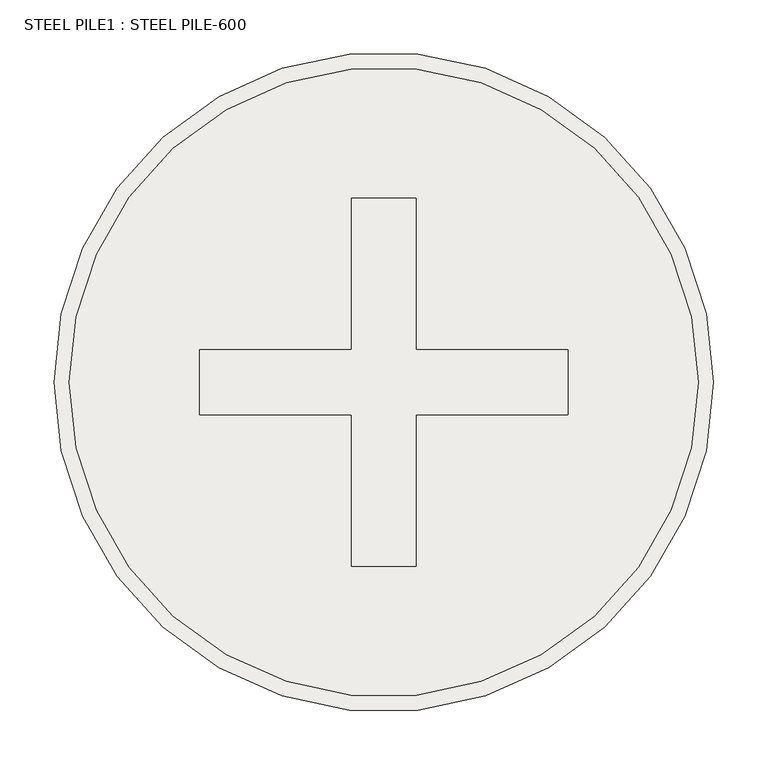
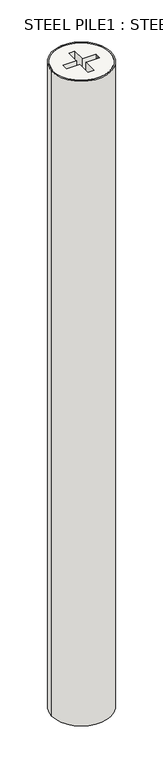
"""IFC4 building model written with IfcOpenShell, lengths in millimetres: slab geometry, STEEL PILE1 : STEEL PILE-600."""

from ifc_helpers import new_model, si_unit, point, frame, frame_2d, origin, place, context, project, spatial, circle_curve, trimmed, segment, composite_curve, outline, extrude, source, transform, mapped, element, save
from ifc_brep_helpers import plane_surface, cylinder_surface, advanced_brep


def steel_pile1_steel_pile_600_91f59ebf(model_context):
    return source(origin(), model_context, "Body", "SolidModel", [
        advanced_brep(
        [(-290.5, 22499.5208589, 150.0), (290.5, 22499.5208589, 150.0), (-30.0, 22469.5208589, 150.0), (-170.0, 22469.5208589, 150.0), (-170.0, 22499.5208589, 150.0), (-170.0, 22529.5208589, 150.0), (-30.0, 22529.5208589, 150.0), (-30.0, 22669.5208589, 150.0), (30.0, 22669.5208589, 150.0), (30.0, 22529.5208589, 150.0), (170.0, 22529.5208589, 150.0), (170.0, 22499.5208589, 150.0), (170.0, 22469.5208589, 150.0), (30.0, 22469.5208589, 150.0), (30.0, 22329.5208589, 150.0), (-30.0, 22329.5208589, 150.0), (-290.5, 22499.5208589, -1850.0), (290.5, 22499.5208589, -1850.0), (-170.0, 22469.5208589, -160.0), (-30.0, 22469.5208589, -160.0), (-30.0, 22329.5208589, -160.0), (30.0, 22329.5208589, -160.0), (30.0, 22469.5208589, -160.0), (170.0, 22469.5208589, -160.0), (170.0, 22499.5208589, -160.0), (170.0, 22529.5208589, -160.0), (30.0, 22529.5208589, -160.0), (30.0, 22669.5208589, -160.0), (-30.0, 22669.5208589, -160.0), (-30.0, 22529.5208589, -160.0), (-170.0, 22529.5208589, -160.0), (-170.0, 22499.5208589, -160.0)],
        [
            (0, 1, circle_curve(frame((0.0, 22499.5208589, 150.0), z_axis=(0.0, 0.0, 1.0), x_axis=(1.0, 0.0, 0.0)), 290.5)),
            (1, 0, circle_curve(frame((0.0, 22499.5208589, 150.0), z_axis=(0.0, 0.0, 1.0), x_axis=(1.0, 0.0, 0.0)), 290.5)),
            (2, 3),
            (3, 4),
            (4, 5),
            (5, 6),
            (6, 7),
            (7, 8),
            (8, 9),
            (9, 10),
            (10, 11),
            (11, 12),
            (12, 13),
            (13, 14),
            (14, 15),
            (15, 2),
            (16, 17, circle_curve(frame((0.0, 22499.5208589, -1850.0), z_axis=(0.0, 0.0, -1.0), x_axis=(1.0, 0.0, 0.0)), 290.5)),
            (17, 16, circle_curve(frame((0.0, 22499.5208589, -1850.0), z_axis=(0.0, 0.0, -1.0), x_axis=(1.0, 0.0, 0.0)), 290.5)),
            (0, 16),
            (17, 1),
            (18, 19),
            (19, 20),
            (20, 21),
            (21, 22),
            (22, 23),
            (23, 24),
            (24, 25),
            (25, 26),
            (26, 27),
            (27, 28),
            (28, 29),
            (29, 30),
            (30, 31),
            (31, 18),
            (18, 3),
            (2, 19),
            (15, 20),
            (14, 21),
            (13, 22),
            (12, 23),
            (11, 24),
            (10, 25),
            (9, 26),
            (8, 27),
            (7, 28),
            (6, 29),
            (5, 30),
            (4, 31),
        ],
        [
            plane_surface(frame((290.5, 22499.5208589, 150.0), z_axis=(0.0, 0.0, 1.0), x_axis=(0.0, 1.0, 0.0))),
            plane_surface(frame((290.5, 22499.5208589, -1850.0), z_axis=(0.0, 0.0, -1.0), x_axis=(0.0, -1.0, 0.0))),
            cylinder_surface(frame((0.0, 22499.5208589, -1850.0), z_axis=(0.0, 0.0, 1.0), x_axis=(1.0, 0.0, 0.0)), 290.5),
            plane_surface(frame((-170.0, 22469.5208589, -160.0), z_axis=(0.0, 0.0, 1.0), x_axis=(-1.0, 0.0, 0.0))),
            plane_surface(frame((-170.0, 22469.5208589, 160.0), z_axis=(0.0, 1.0, 0.0), x_axis=(0.0, 0.0, -1.0))),
            plane_surface(frame((-30.0, 22469.5208589, 160.0), z_axis=(1.0, 0.0, 0.0), x_axis=(0.0, 0.0, -1.0))),
            plane_surface(frame((-30.0, 22329.5208589, 160.0), z_axis=(0.0, 1.0, 0.0), x_axis=(0.0, 0.0, -1.0))),
            plane_surface(frame((30.0, 22329.5208589, 160.0), z_axis=(-1.0, 0.0, 0.0), x_axis=(0.0, 0.0, -1.0))),
            plane_surface(frame((30.0, 22469.5208589, 160.0), z_axis=(0.0, 1.0, 0.0), x_axis=(0.0, 0.0, -1.0))),
            plane_surface(frame((170.0, 22469.5208589, 160.0), z_axis=(-1.0, 0.0, 0.0), x_axis=(0.0, 0.0, -1.0))),
            plane_surface(frame((170.0, 22499.5208589, 160.0), z_axis=(-1.0, 0.0, 0.0), x_axis=(0.0, 0.0, -1.0))),
            plane_surface(frame((170.0, 22529.5208589, 160.0), z_axis=(0.0, -1.0, 0.0), x_axis=(0.0, 0.0, -1.0))),
            plane_surface(frame((30.0, 22529.5208589, 160.0), z_axis=(-1.0, 0.0, 0.0), x_axis=(0.0, 0.0, -1.0))),
            plane_surface(frame((30.0, 22669.5208589, 160.0), z_axis=(0.0, -1.0, 0.0), x_axis=(0.0, 0.0, -1.0))),
            plane_surface(frame((-30.0, 22669.5208589, 160.0), z_axis=(1.0, 0.0, 0.0), x_axis=(0.0, 0.0, -1.0))),
            plane_surface(frame((-30.0, 22529.5208589, 160.0), z_axis=(0.0, -1.0, 0.0), x_axis=(0.0, 0.0, -1.0))),
            plane_surface(frame((-170.0, 22529.5208589, 160.0), z_axis=(1.0, 0.0, 0.0), x_axis=(0.0, 0.0, -1.0))),
            plane_surface(frame((-170.0, 22499.5208589, 160.0), z_axis=(1.0, 0.0, 0.0), x_axis=(0.0, 0.0, -1.0))),
        ],
        [
            (0, [[1, 2], [3, 4, 5, 6, 7, 8, 9, 10, 11, 12, 13, 14, 15, 16]]),
            (1, [[17, 18]]),
            (2, [[-1, 19, -18, 20]]),
            (2, [[-2, -20, -17, -19]]),
            (3, [[21, 22, 23, 24, 25, 26, 27, 28, 29, 30, 31, 32, 33, 34]]),
            (4, [[-21, 35, -3, 36]]),
            (5, [[-22, -36, -16, 37]]),
            (6, [[-23, -37, -15, 38]]),
            (7, [[-24, -38, -14, 39]]),
            (8, [[-25, -39, -13, 40]]),
            (9, [[-26, -40, -12, 41]]),
            (10, [[-27, -41, -11, 42]]),
            (11, [[-28, -42, -10, 43]]),
            (12, [[-29, -43, -9, 44]]),
            (13, [[-30, -44, -8, 45]]),
            (14, [[-31, -45, -7, 46]]),
            (15, [[-32, -46, -6, 47]]),
            (16, [[-33, -47, -5, 48]]),
            (17, [[-34, -48, -4, -35]]),
        ],
    ),
        extrude(outline(composite_curve([segment(trimmed(circle_curve(frame_2d((0.0, 22499.5208589)), 304.5), [point((-304.5, 22499.5208589))], [point((304.5, 22499.5208589))], False, "CARTESIAN"), True, "CONTINUOUS"), segment(trimmed(circle_curve(frame_2d((0.0, 22499.5208589)), 304.5), [point((304.5, 22499.5208589))], [point((-304.5, 22499.5208589))], False, "CARTESIAN"), True, "CONTINUOUS")], self_intersect=False), holes=[composite_curve([segment(trimmed(circle_curve(frame_2d((0.0, 22499.5208589)), 290.5), [point((-290.5, 22499.5208589))], [point((290.5, 22499.5208589))], True, "CARTESIAN"), True, "CONTINUOUS"), segment(trimmed(circle_curve(frame_2d((0.0, 22499.5208589)), 290.5), [point((290.5, 22499.5208589))], [point((-290.5, 22499.5208589))], True, "CARTESIAN"), True, "CONTINUOUS")], self_intersect=False)]), frame((0.0, 0.0, -6850.0), z_axis=(0.0, 0.0, 1.0), x_axis=(1.0, 0.0, 0.0)), (0.0, 0.0, 1.0), 7000.0),
    ])


if __name__ == "__main__":
    model = new_model("IFC4")
    model_context = context("Model", 3, world=origin())
    ifc_project = project(units=[si_unit("LENGTHUNIT", "METRE", prefix="MILLI")], contexts=[model_context])
    site = spatial("IfcSite", under=ifc_project)
    building = spatial("IfcBuilding", under=site)
    placement = place(None, origin())
    steel_pile1_steel_pile_600_shape = steel_pile1_steel_pile_600_91f59ebf(model_context)
    element("IfcSlab", 1, ObjectType="STEEL PILE1 : STEEL PILE-600", at=placement, inside=building, context=model_context, shape_type="MappedRepresentation", body=[
        mapped(steel_pile1_steel_pile_600_shape, transform((0.0, 0.0, 0.0), x_axis=(1.0, 0.0, 0.0), y_axis=(0.0, 1.0, 0.0), z_axis=(0.0, 0.0, 1.0))),
    ])
    save(model, "model.ifc")
